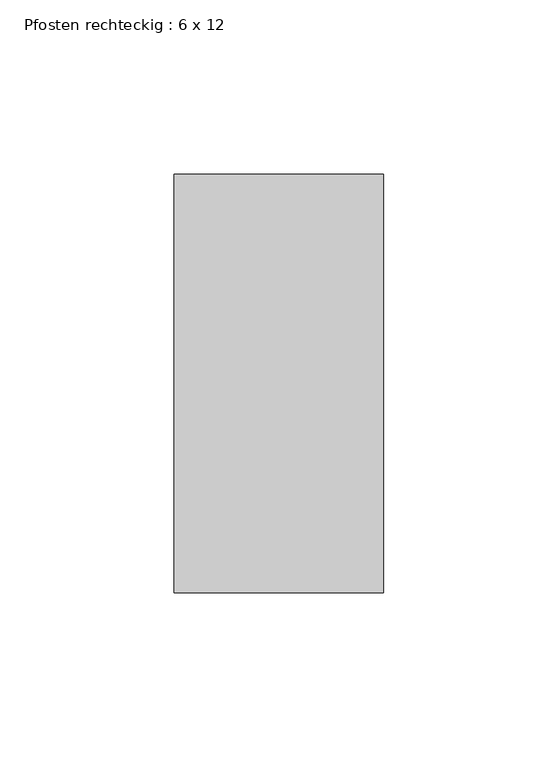
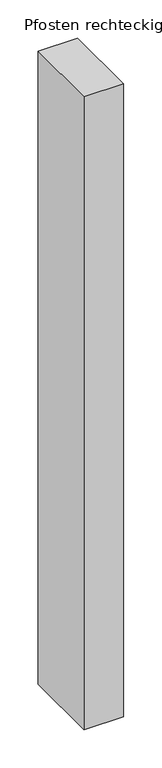
"""IFC4 building model written with IfcOpenShell, lengths in millimetres: member geometry, Pfosten rechteckig : 6 x 12."""

from ifc_helpers import new_model, si_unit, frame, origin, place, context, project, spatial, polyline, outline, extrude, source, transform, mapped, element, save


def pfosten_rechteckig_6_x_12_c0675010(model_context):
    return source(origin(), model_context, "Body", "SweptSolid", [
        extrude(outline(polyline([(30.0, 60.0), (30.0, -60.0), (-30.0, -60.0), (-30.0, 60.0), (30.0, 60.0)])), frame((0.0, 0.0, -1009.9773049), z_axis=(0.0, 0.0, 1.0), x_axis=(1.0, 0.0, 0.0)), (0.0, 0.0, 1.0), 1009.9773049),
    ])


if __name__ == "__main__":
    model = new_model("IFC4")
    model_context = context("Model", 3, world=origin())
    ifc_project = project(units=[si_unit("LENGTHUNIT", "METRE", prefix="MILLI")], contexts=[model_context])
    site = spatial("IfcSite", under=ifc_project)
    building = spatial("IfcBuilding", under=site)
    placement = place(None, origin())
    pfosten_rechteckig_6_x_12_shape = pfosten_rechteckig_6_x_12_c0675010(model_context)
    element("IfcMember", 1, ObjectType="Pfosten rechteckig : 6 x 12", at=placement, inside=building, context=model_context, shape_type="MappedRepresentation", body=[
        mapped(pfosten_rechteckig_6_x_12_shape, transform((0.0, 0.0, 0.0), x_axis=(1.0, 0.0, 0.0), y_axis=(0.0, 1.0, 0.0), z_axis=(0.0, 0.0, 1.0))),
    ])
    save(model, "model.ifc")

# Revit data of these elements
# Type "Pfosten rechteckig : 6 x 12"
#   built-in parameter 1007304 = 0.393701 (stored number, unit not read)
#   built-in parameter 1007301 = 0.0984252 (stored number, unit not read)
#   built-in parameter 1007300 = 0.0984252 (stored number, unit not read)
# Element 1 (IfcMember, "Pfosten rechteckig : 6 x 12")
#   Materials on its faces: "Metall - verzinkt"
# Materials
#   "Metall - verzinkt": class "Allgemeines", colour RGB 200 200 200, transparency 0, Cost = 0
